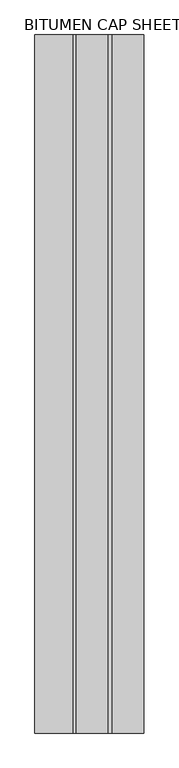
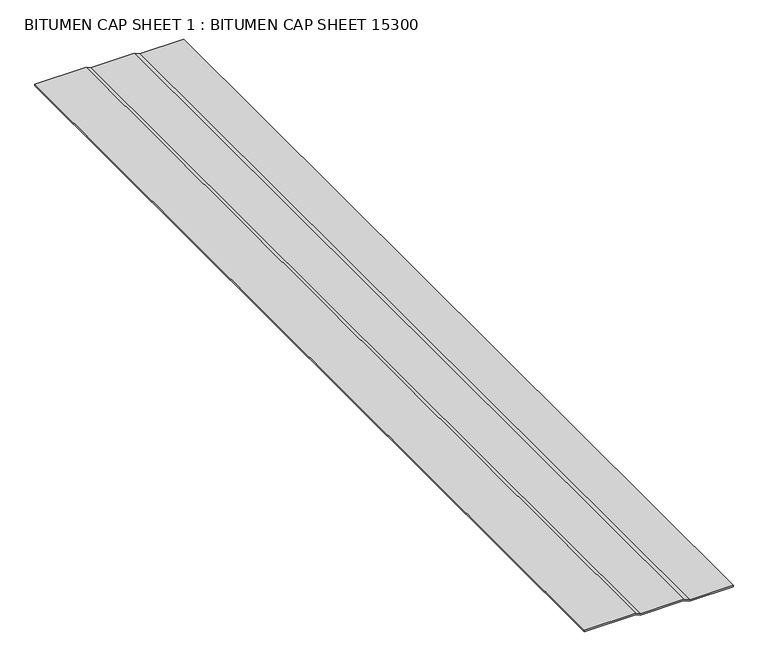
"""IFC4 building model written with IfcOpenShell, lengths in millimetres: proxy geometry, BITUMEN CAP SHEET 1 : BITUMEN CAP SHEET 15300."""

from ifc_helpers import new_model, si_unit, frame, origin, place, context, project, spatial, polyline, outline, extrude, source, transform, mapped, element, save


def bitumen_cap_sheet_1_bitumen_cap_sheet_15300_313e2dc3(model_context):
    return source(origin(), model_context, "Body", "SweptSolid", [
        extrude(outline(polyline([(40259.2002678, -2469.2761954), (40262.3752678, -2469.2761954), (40262.3752678, -2560.795457), (40267.6612773, -2573.2602756), (40267.6612773, -2663.9440313), (40271.9940719, -2673.6609328), (40271.9940719, -2781.5474293), (40268.8188423, -2781.5474293), (40268.8188423, -2674.3362183), (40264.4862773, -2664.6198318), (40264.4862773, -2573.9056756), (40259.2002678, -2561.440857), (40259.2002678, -2469.2761954)])), frame((0.0, -1052.8906574, 0.0), z_axis=(0.0, 1.0, 0.0), x_axis=(0.0, 0.0, 1.0)), (0.0, 0.0, 1.0), 2000.25),
    ])


if __name__ == "__main__":
    model = new_model("IFC4")
    model_context = context("Model", 3, world=origin())
    ifc_project = project(units=[si_unit("LENGTHUNIT", "METRE", prefix="MILLI")], contexts=[model_context])
    site = spatial("IfcSite", under=ifc_project)
    building = spatial("IfcBuilding", under=site)
    placement = place(None, origin())
    bitumen_cap_sheet_1_bitumen_cap_sheet_15300_shape = bitumen_cap_sheet_1_bitumen_cap_sheet_15300_313e2dc3(model_context)
    element("IfcBuildingElementProxy", 1, Name="BITUMEN CAP SHEET 1 : BITUMEN CAP SHEET 15300", ObjectType="BITUMEN CAP SHEET 1 : BITUMEN CAP SHEET 15300", at=placement, inside=building, context=model_context, shape_type="MappedRepresentation", body=[
        mapped(bitumen_cap_sheet_1_bitumen_cap_sheet_15300_shape, transform((0.0, 0.0, 0.0), x_axis=(1.0, 0.0, 0.0), y_axis=(0.0, 1.0, 0.0), z_axis=(0.0, 0.0, 1.0))),
    ])
    save(model, "model.ifc")

# Revit data of these elements
# Type "BITUMEN CAP SHEET 1 : BITUMEN CAP SHEET 15300"
#   NameOverride = "BITUMEN CAP SHEET"
# Element 1 (IfcBuildingElementProxy, "BITUMEN CAP SHEET 1 : BITUMEN CAP SHEET 15300")
#   Materials on its faces: "MODIFIED BITUMEN GRANULE SURFACED CAP SHEET"
# Materials
#   "MODIFIED BITUMEN GRANULE SURFACED CAP SHEET": class "Unassigned", colour RGB 85 85 127, transparency 0
